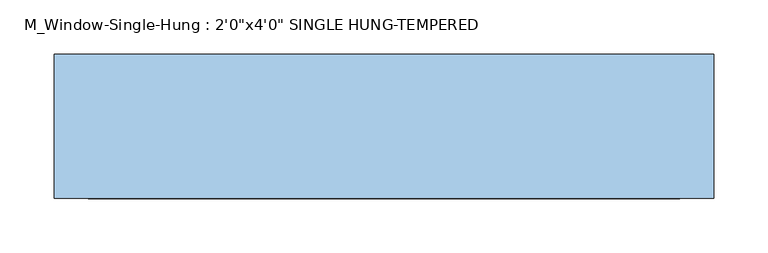
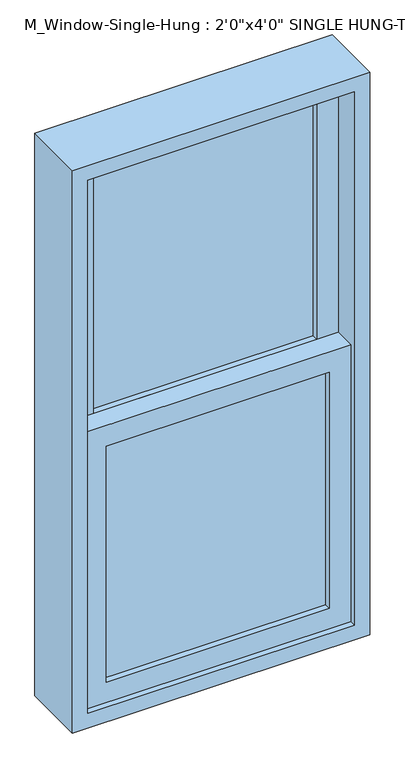
"""IFC4 building model written with IfcOpenShell, lengths in millimetres: window geometry."""

from ifc_helpers import new_model, si_unit, frame, origin, place, context, project, spatial, polyline, outline, extrude, source, transform, mapped, element, save


def window_3f32ae63(model_context):
    return source(origin(), model_context, "Body", "SweptSolid", [
        extrude(outline(polyline([(228.6, -19.05), (228.6, -25.4), (-228.6, -25.4), (-228.6, -19.05), (228.6, -19.05)])), frame((0.0, 0.0, 990.6), z_axis=(0.0, 0.0, 1.0), x_axis=(1.0, 0.0, 0.0)), (0.0, 0.0, 1.0), 511.175),
        extrude(outline(polyline([(-228.6, -31.75), (228.6, -31.75), (228.6, -38.1), (-228.6, -38.1), (-228.6, -31.75)])), frame((0.0, 0.0, 990.6), z_axis=(0.0, 0.0, 1.0), x_axis=(1.0, 0.0, 0.0)), (0.0, 0.0, 1.0), 511.175),
        extrude(outline(polyline([(228.6, 25.4), (228.6, 19.05), (-228.6, 19.05), (-228.6, 25.4), (228.6, 25.4)])), frame((0.0, 0.0, 1546.225), z_axis=(0.0, 0.0, 1.0), x_axis=(1.0, 0.0, 0.0)), (0.0, 0.0, 1.0), 511.175),
        extrude(outline(polyline([(-228.6, 12.7), (228.6, 12.7), (228.6, 6.35), (-228.6, 6.35), (-228.6, 12.7)])), frame((0.0, 0.0, 1546.225), z_axis=(0.0, 0.0, 1.0), x_axis=(1.0, 0.0, 0.0)), (0.0, 0.0, 1.0), 511.175),
        extrude(outline(polyline([(1546.225, -273.05), (946.15, -273.05), (946.15, 273.05), (1546.225, 273.05), (1546.225, -273.05)]), holes=[polyline([(1501.775, 228.6), (990.6, 228.6), (990.6, -228.6), (1501.775, -228.6), (1501.775, 228.6)])]), frame((0.0, -50.8, 0.0), z_axis=(0.0, 1.0, 0.0), x_axis=(0.0, 0.0, 1.0)), (0.0, 0.0, 1.0), 44.45),
        extrude(outline(polyline([(2101.85, -273.05), (1501.775, -273.05), (1501.775, 273.05), (2101.85, 273.05), (2101.85, -273.05)]), holes=[polyline([(2057.4, 228.6), (1546.225, 228.6), (1546.225, -228.6), (2057.4, -228.6), (2057.4, 228.6)])]), frame((0.0, -6.35, 0.0), z_axis=(0.0, 1.0, 0.0), x_axis=(0.0, 0.0, 1.0)), (0.0, 0.0, 1.0), 44.45),
        extrude(outline(polyline([(2133.6, -304.8), (914.4, -304.8), (914.4, 304.8), (2133.6, 304.8), (2133.6, -304.8)]), holes=[polyline([(2101.85, 273.05), (946.15, 273.05), (946.15, -273.05), (2101.85, -273.05), (2101.85, 273.05)])]), frame((0.0, -63.5, 0.0), z_axis=(0.0, 1.0, 0.0), x_axis=(0.0, 0.0, 1.0)), (0.0, 0.0, 1.0), 133.35),
    ])


if __name__ == "__main__":
    model = new_model("IFC4")
    model_context = context("Model", 3, world=origin())
    ifc_project = project(units=[si_unit("LENGTHUNIT", "METRE", prefix="MILLI")], contexts=[model_context])
    site = spatial("IfcSite", under=ifc_project)
    building = spatial("IfcBuilding", under=site)
    placement = place(None, origin())
    window_shape = window_3f32ae63(model_context)
    element("IfcWindow", 1, ObjectType="M_Window-Single-Hung : 2'0\"x4'0\" SINGLE HUNG-TEMPERED", at=placement, inside=building, context=model_context, shape_type="MappedRepresentation", body=[
        mapped(window_shape, transform((0.0, 0.0, 0.0), x_axis=(1.0, 0.0, 0.0), y_axis=(0.0, 1.0, 0.0), z_axis=(0.0, 0.0, 1.0))),
    ])
    save(model, "model.ifc")

# Revit data of these elements
# Type "M_Window-Single-Hung : 2'0\"x4'0\" SINGLE HUNG-TEMPERED"
#   Type Mark = "2"
#   Fire Rating = "0.5h"
#   Construction Type Id = "DG-DR"
#   Assembly Code = "B2020100"
#   Analytic Construction = "Double glazing - domestic"
#   Wall Thickness [instance default] = 0' - 5.90551"
#   Window Inset [instance default] = 0' - 0"
#   Visual Light Transmittance = 0.81
#   Thermal Resistance (R) = 1.8146 (h·ft²·°F)/BTU
#   Solar Heat Gain Coefficient = 0.76
#   Muntin Width = 1' - 6"
#   Muntin Height = 1' - 8 1/8"
#   Interior Wall Closure [instance default] = 0' - 1.40551"
#   Rough Width = 2' - 0.59055"
#   Rough Height = 4' - 0.59055"
#   Frame Extension [instance default] = 0' - 1 1/4"
#   Exterior Wall Closure [instance default] = 0' - 0 1/2"
#   Extension Jamb [instance default] = 0' - 1.40551"
#   Heat Transfer Coefficient (U) = 0.5511 BTU/(h·ft²·°F)
#   Height = 4' - 0"
#   Width = 2' - 0"
#   Top Muntin Visibility = yes
#   Indicator Visibility [instance default] = yes
#   Extension Jamb Visibility [instance default] = yes
#   Interior Trim Visibility [instance default] = yes
#   Exterior Trim Visibility [instance default] = yes
#   Define Thermal Properties by = 1
#   Bottom Muntin Visibility = yes
#   Muntin Pattern = M_Muntin Pattern_2x2 : M_Muntin Pattern_2x2
#   Interior Trim Material = Wood - Stained
#   Interior Trim = M_Trim-Window-Interior-Flat : Picture Frame
#   Exterior Trim Material = Clad - White
#   Exterior Trim = M_Trim-Window-Exterior-Flat : with Sill
#   Glass Panel Material = Glass
#   Exterior Frame Material = Clad - White
#   Interior Frame Material = Wood - Stained
#   Wall Closure = (empty or 0)
# Element 1 (IfcWindow, "M_Window-Single-Hung : 2'0\"x4'0\" SINGLE HUNG-TEMPERED")
#   Wall Thickness = 0' - 4"
#   Extension Jamb = 0' - 1"
#   Extension Jamb Visibility = no
#   Materials on its faces: "Wood - Stained", "Glass", "Clad - White"
# Materials
#   "Wood - Stained": class "Wood", colour RGB 224 178 126, transparency 0, Cost = 0
#   "Clad - White": class "Wood", colour RGB 242 242 238, transparency 0, Cost = 0
#   "Glass": class "Glass", colour RGB 0 128 192, transparency 0.75, Description = "Soda Lime Glass", Cost = 0
